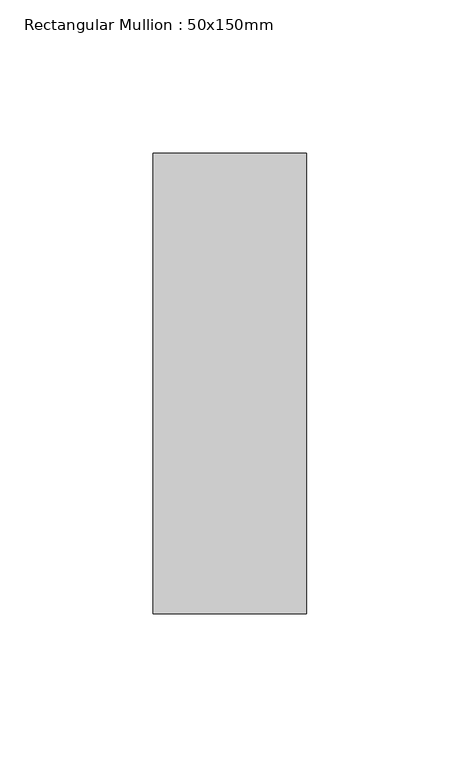
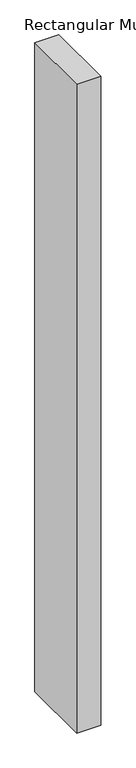
"""IFC4 building model written with IfcOpenShell, lengths in millimetres: member geometry, Rectangular Mullion : 50x150mm."""

from ifc_helpers import new_model, si_unit, frame, origin, place, context, project, spatial, polyline, outline, extrude, source, transform, mapped, element, save


def rectangular_mullion_50x150mm_acb4c03f(model_context):
    return source(origin(), model_context, "Body", "SweptSolid", [
        extrude(outline(polyline([(25.0, 75.0), (25.0, -75.0), (-25.0, -75.0), (-25.0, 75.0), (25.0, 75.0)])), frame((0.0, 0.0, -1425.0000002), z_axis=(0.0, 0.0, 1.0), x_axis=(1.0, 0.0, 0.0)), (0.0, 0.0, 1.0), 1425.0000002),
    ])


if __name__ == "__main__":
    model = new_model("IFC4")
    model_context = context("Model", 3, world=origin())
    ifc_project = project(units=[si_unit("LENGTHUNIT", "METRE", prefix="MILLI")], contexts=[model_context])
    site = spatial("IfcSite", under=ifc_project)
    building = spatial("IfcBuilding", under=site)
    placement = place(None, origin())
    rectangular_mullion_50x150mm_shape = rectangular_mullion_50x150mm_acb4c03f(model_context)
    element("IfcMember", 1, ObjectType="Rectangular Mullion : 50x150mm", at=placement, inside=building, context=model_context, shape_type="MappedRepresentation", body=[
        mapped(rectangular_mullion_50x150mm_shape, transform((0.0, 0.0, 0.0), x_axis=(1.0, 0.0, 0.0), y_axis=(0.0, 1.0, 0.0), z_axis=(0.0, 0.0, 1.0))),
    ])
    save(model, "model.ifc")

# Revit data of these elements
# Type "Rectangular Mullion : 50x150mm"
#   Keynote = "H11"
#   built-in parameter 1007304 = 0.492126 (stored number, unit not read)
#   built-in parameter 1007301 = 0.082021 (stored number, unit not read)
#   built-in parameter 1007300 = 0.082021 (stored number, unit not read)
# Element 1 (IfcMember, "Rectangular Mullion : 50x150mm")
#   Materials on its faces: "Aluminium"
# Materials
#   "Aluminium": class "Metal", colour RGB 247 247 247, transparency 0, Description = "Aluminium 6061", Cost = 0
